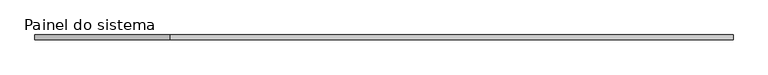
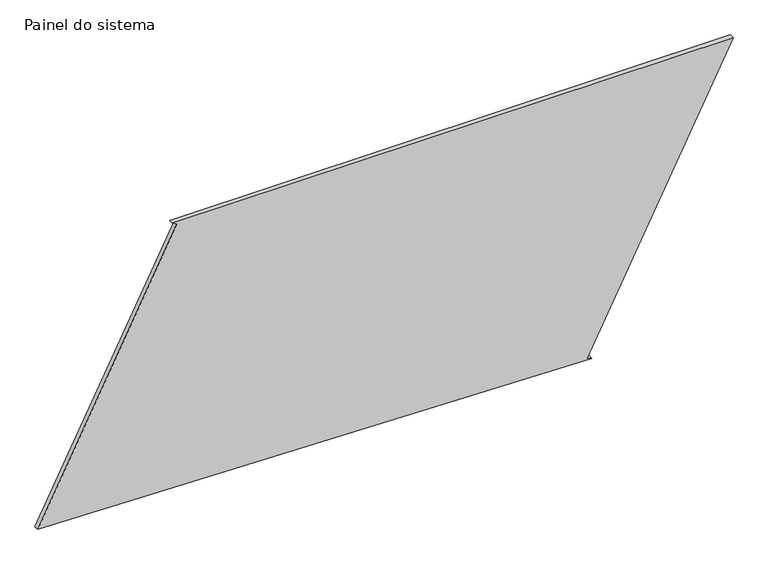
"""IFC4 building model written with IfcOpenShell, lengths in millimetres: plate geometry, Painel do sistema : Envidraçado."""

from ifc_helpers import new_model, si_unit, frame, origin, place, context, project, spatial, polyline, outline, extrude, source, transform, mapped, element, save


def painel_do_sistema_a1723807(model_context):
    return source(origin(), model_context, "Body", "SweptSolid", [
        extrude(outline(polyline([(0.0, 1051.3830352), (11.291819, 1029.0784432), (1476.5355055, 1770.8658938), (1476.5355055, -1084.6323567), (1465.2436865, -1062.3277647), (65.6769784, -1770.8658938), (0.0, 1051.3830352)])), frame((0.0, 24.5, 0.0), z_axis=(0.0, 1.0, 0.0), x_axis=(0.0, 0.0, 1.0)), (0.0, 0.0, 1.0), 25.0),
    ])


if __name__ == "__main__":
    model = new_model("IFC4")
    model_context = context("Model", 3, world=origin())
    ifc_project = project(units=[si_unit("LENGTHUNIT", "METRE", prefix="MILLI")], contexts=[model_context])
    site = spatial("IfcSite", under=ifc_project)
    building = spatial("IfcBuilding", under=site)
    placement = place(None, origin())
    painel_do_sistema_shape = painel_do_sistema_a1723807(model_context)
    element("IfcPlate", 1, ObjectType="Painel do sistema : Envidraçado", at=placement, inside=building, context=model_context, shape_type="MappedRepresentation", body=[
        mapped(painel_do_sistema_shape, transform((0.0, 0.0, 0.0), x_axis=(1.0, 0.0, 0.0), y_axis=(0.0, 1.0, 0.0), z_axis=(0.0, 0.0, 1.0))),
    ])
    save(model, "model.ifc")

# Revit data of these elements
# Type "Painel do sistema : Envidraçado"
#   Construction Type Id = "GSP4R"
#   Analytic Construction = "Vidraça única Pilkington 1/8 pol"
#   Visual Light Transmittance = 0.9
#   Solar Heat Gain Coefficient = 0.86
#   Heat Transfer Coefficient (U) = 6.7069 W/(m²·K)
# Element 1 (IfcPlate, "Painel do sistema : Envidraçado")
#   Materials on its faces: "Vidro"
# Materials
#   "Vidro": class "Vidro", colour RGB 0 128 192, transparency 0.9, Description = "Vidro de sílica", Cost = 0
